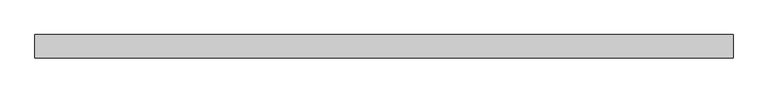
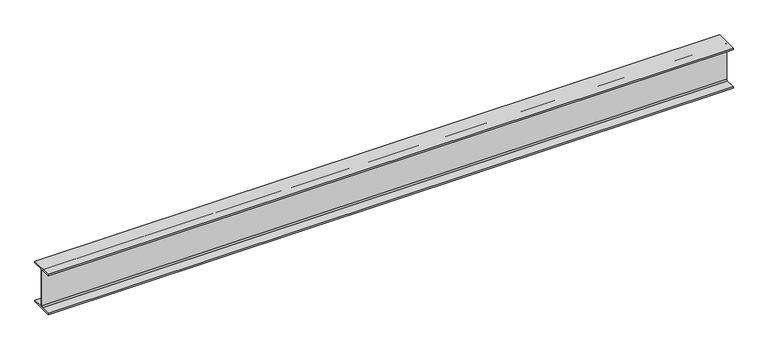
"""IFC4 building model written with IfcOpenShell, lengths in millimetres: beam geometry, Steel Beam_H-KSD3502 : H_SB_ASB_H-300x300x10x15."""

import ifcopenshell
import ifcopenshell.guid

model = None  # the IFC model being written
_history = None  # IfcOwnerHistory: only IFC2X3 demands one
_inside = {}  # id of a spatial element -> (the spatial element, [elements in it])
_under = {}  # id of a project, library or spatial element -> (it, [spatial elements below it])
_declared = {}  # id of a project -> (the project, [libraries it declares])
_typed = {}  # id of a type object -> (the type object, [elements of that type])
_made_of = {}  # id of a material, layer set ... -> (it, [elements and type objects made of it])


def new_model(schema):
    """Start an empty IFC model of exactly this schema.

    Asked for "IFC4X3", IfcOpenShell would pick the latest addendum, in which some entities
    have other attributes; the version numbers below select the first issue.
    IFC2X3 requires an IfcOwnerHistory on every rooted entity: one is made here for all.
    """
    global model, _history
    if schema == "IFC4X3":
        model = ifcopenshell.file(schema_version=(4, 3, 0, 0))
    else:
        model = ifcopenshell.file(schema=schema)
    _inside.clear()
    _under.clear()
    _declared.clear()
    _typed.clear()
    _made_of.clear()
    _history = None
    if model.schema == "IFC2X3":
        org = make("IfcOrganization", Name="unknown")
        user = make(
            "IfcPersonAndOrganization",
            ThePerson=make("IfcPerson", FamilyName="unknown"),
            TheOrganization=org,
        )
        app = make(
            "IfcApplication",
            ApplicationDeveloper=org,
            Version="unknown",
            ApplicationFullName="unknown",
            ApplicationIdentifier="unknown",
        )
        _history = make(
            "IfcOwnerHistory",
            OwningUser=user,
            OwningApplication=app,
            ChangeAction="ADDED",
            CreationDate=0,
        )
    return model


def make(cls, **values):
    """One entity of the class cls with the attributes given. An attribute that is None is left unset."""
    return model.create_entity(
        cls, **{name: value for name, value in values.items() if value is not None}
    )


def rooted(cls, **values):
    """An entity with a GlobalId (a new one), such as an element, a storey or a relation."""
    return make(cls, GlobalId=ifcopenshell.guid.new(), OwnerHistory=_history, **values)


def si_unit(unit_type, name, prefix=None):
    """IfcSIUnit, for example si_unit("LENGTHUNIT", "METRE", prefix="MILLI")."""
    return make("IfcSIUnit", UnitType=unit_type, Prefix=prefix, Name=name)


def assignment(units):
    """IfcUnitAssignment: the units of a project."""
    return None if units is None else make("IfcUnitAssignment", Units=units)


def point(xyz):
    """IfcCartesianPoint."""
    return None if xyz is None else make("IfcCartesianPoint", Coordinates=xyz)


def direction(xyz):
    """IfcDirection."""
    return None if xyz is None else make("IfcDirection", DirectionRatios=xyz)


def frame(location, z_axis=None, x_axis=None):
    """IfcAxis2Placement3D, a coordinate frame: its origin and axes. An axis left out is left unset."""
    return make(
        "IfcAxis2Placement3D",
        Location=point(location),
        Axis=direction(z_axis),
        RefDirection=direction(x_axis),
    )


def frame_2d(location, x_axis=None):
    """IfcAxis2Placement2D, a coordinate frame in the plane: its origin and x axis."""
    return make(
        "IfcAxis2Placement2D", Location=point(location), RefDirection=direction(x_axis)
    )


def origin():
    """The frame at (0, 0, 0) with its axes left unset."""
    return frame((0.0, 0.0, 0.0))


def place(relative_to, where):
    """IfcLocalPlacement: puts the frame where relative to a parent placement (None: the world)."""
    return make(
        "IfcLocalPlacement", PlacementRelTo=relative_to, RelativePlacement=where
    )


def context(
    kind, dimensions, precision=None, world=None, true_north=None, identifier=None
):
    """IfcGeometricRepresentationContext, for example the 3D "Model" context."""
    return make(
        "IfcGeometricRepresentationContext",
        ContextIdentifier=identifier,
        ContextType=kind,
        CoordinateSpaceDimension=dimensions,
        Precision=precision,
        WorldCoordinateSystem=world,
        TrueNorth=true_north,
    )


def project(units=None, contexts=None):
    """IfcProject with its units and contexts."""
    return rooted(
        "IfcProject",
        Name="project",
        RepresentationContexts=contexts,
        UnitsInContext=assignment(units),
    )


def spatial(cls, under=None, at=None, **own):
    """A site, building, storey or space (cls), placed at a placement, below another one or the project."""
    s = rooted(cls, ObjectPlacement=at, **own)
    if under is not None:
        _under.setdefault(under.id(), (under, []))[1].append(s)
    return s


def polyline(points):
    """IfcPolyline through the points."""
    return make("IfcPolyline", Points=[point(p) for p in points])


def circle_curve(where, radius):
    """IfcCircle in the frame where."""
    return make("IfcCircle", Position=where, Radius=radius)


def trimmed(basis, trim1, trim2, sense, master):
    """IfcTrimmedCurve: the piece of a basis curve between two trims."""
    return make(
        "IfcTrimmedCurve",
        BasisCurve=basis,
        Trim1=trim1,
        Trim2=trim2,
        SenseAgreement=sense,
        MasterRepresentation=master,
    )


def segment(curve, same_sense, transition):
    """IfcCompositeCurveSegment."""
    return make(
        "IfcCompositeCurveSegment",
        Transition=transition,
        SameSense=same_sense,
        ParentCurve=curve,
    )


def composite_curve(segments, self_intersect=None):
    """IfcCompositeCurve: segments joined end to end."""
    return make("IfcCompositeCurve", Segments=segments, SelfIntersect=self_intersect)


def outline(outer, holes=None, kind="AREA"):
    """IfcArbitraryClosedProfileDef: a profile drawn as a closed curve; with holes, ...WithVoids."""
    if holes is None:
        return make("IfcArbitraryClosedProfileDef", ProfileType=kind, OuterCurve=outer)
    return make(
        "IfcArbitraryProfileDefWithVoids",
        ProfileType=kind,
        OuterCurve=outer,
        InnerCurves=holes,
    )


def extrude(swept, where, along, depth):
    """IfcExtrudedAreaSolid: the profile swept, set in the frame where, extruded along a direction by depth."""
    return make(
        "IfcExtrudedAreaSolid",
        SweptArea=swept,
        Position=where,
        ExtrudedDirection=direction(along),
        Depth=depth,
    )


def shape(context_of_items, identifier, shape_type, items):
    """IfcShapeRepresentation: the items that make up one representation, for example the "Body"."""
    return make(
        "IfcShapeRepresentation",
        ContextOfItems=context_of_items,
        RepresentationIdentifier=identifier,
        RepresentationType=shape_type,
        Items=items,
    )


def source(mapping_origin, context_of_items, identifier, shape_type, items):
    """IfcRepresentationMap: a shape defined once, which mapped items show again and again."""
    return make(
        "IfcRepresentationMap",
        MappingOrigin=mapping_origin,
        MappedRepresentation=shape(context_of_items, identifier, shape_type, items),
    )


def transform(
    local_origin,
    x_axis=None,
    y_axis=None,
    z_axis=None,
    scale=None,
    scale2=None,
    scale3=None,
    uniform=True,
):
    """IfcCartesianTransformationOperator3D, or its non-uniform kind. x_axis, y_axis, z_axis: its Axis1, 2, 3."""
    if uniform:
        return make(
            "IfcCartesianTransformationOperator3D",
            Axis1=direction(x_axis),
            Axis2=direction(y_axis),
            LocalOrigin=point(local_origin),
            Scale=scale,
            Axis3=direction(z_axis),
        )
    return make(
        "IfcCartesianTransformationOperator3DnonUniform",
        Axis1=direction(x_axis),
        Axis2=direction(y_axis),
        LocalOrigin=point(local_origin),
        Scale=scale,
        Axis3=direction(z_axis),
        Scale2=scale2,
        Scale3=scale3,
    )


def mapped(mapping_source, mapping_target):
    """IfcMappedItem: shows the shape of a source again, moved by a transform."""
    return make(
        "IfcMappedItem", MappingSource=mapping_source, MappingTarget=mapping_target
    )


def made_of(thing, what):
    """Note that an element or type object is made of a material, layer set ...; save() writes the relation."""
    if what is not None:
        _made_of.setdefault(what.id(), (what, []))[1].append(thing)
    return thing


def element(
    cls,
    number,
    at=None,
    inside=None,
    cuts=None,
    type_object=None,
    material=None,
    context=None,
    identifier="Body",
    shape_type=None,
    held_by="IfcProductDefinitionShape",
    body=None,
    shapes=None,
    **own,
):
    """One element of the class cls, such as IfcWall. Its Tag is "e" and its number.

    at: its placement. inside: the storey or other place that contains it. cuts: it is an
    opening in that element (IfcRelVoidsElement). A single representation is given by context,
    identifier, shape_type and body (its items); several are given by shapes. held_by: the class
    of the entity that holds the representations. save() writes the other relations.
    """
    e = rooted(cls, Tag="e%d" % number, ObjectPlacement=at, **own)
    if body is not None:
        shapes = [shape(context, identifier, shape_type, body)]
    if shapes is not None:
        e.Representation = make(held_by, Representations=shapes)
    if inside is not None:
        _inside.setdefault(inside.id(), (inside, []))[1].append(e)
    if cuts is not None:
        rooted(
            "IfcRelVoidsElement", RelatingBuildingElement=cuts, RelatedOpeningElement=e
        )
    if type_object is not None:
        _typed.setdefault(type_object.id(), (type_object, []))[1].append(e)
    return made_of(e, material)


def aggregate(whole, parts):
    """IfcRelAggregates: a whole, such as a stair, and the parts it consists of."""
    return rooted("IfcRelAggregates", RelatingObject=whole, RelatedObjects=parts)


def save(model, path):
    """Write the relations noted so far, then the file.

    IfcRelAggregates (storeys below a building ...), IfcRelContainedInSpatialStructure (elements
    in a storey), IfcRelDefinesByType, IfcRelAssociatesMaterial and IfcRelDeclares: one each for
    every whole, place, type object, material and project.
    """
    for whole, parts in _under.values():
        aggregate(whole, parts)
    for where, things in _inside.values():
        rooted(
            "IfcRelContainedInSpatialStructure",
            RelatedElements=things,
            RelatingStructure=where,
        )
    for kind, things in _typed.values():
        rooted("IfcRelDefinesByType", RelatedObjects=things, RelatingType=kind)
    for what, things in _made_of.values():
        rooted("IfcRelAssociatesMaterial", RelatedObjects=things, RelatingMaterial=what)
    for by, libraries in _declared.values():
        rooted("IfcRelDeclares", RelatingContext=by, RelatedDefinitions=libraries)
    model.write(path)


def beam_952dd806(model_context):
    return source(origin(), model_context, "Body", "SweptSolid", [
        extrude(outline(composite_curve([segment(polyline([(-82.5, -141.5), (-11.9, -141.5)]), True, "CONTINUOUS"), segment(trimmed(circle_curve(frame_2d((-11.9, -132.6)), 8.9), [point((-11.9, -141.5))], [point((-3.0, -132.6))], True, "CARTESIAN"), True, "CONTINUOUS"), segment(polyline([(-3.0, -132.6), (-3.0, 132.6)]), True, "CONTINUOUS"), segment(trimmed(circle_curve(frame_2d((-11.9, 132.6)), 8.9), [point((-3.0, 132.6))], [point((-11.9, 141.5))], True, "CARTESIAN"), True, "CONTINUOUS"), segment(polyline([(-11.9, 141.5), (-82.5, 141.5), (-82.5, 151.7), (82.5, 151.7), (82.5, 141.5), (11.9, 141.5)]), True, "CONTINUOUS"), segment(trimmed(circle_curve(frame_2d((11.9, 132.6)), 8.9), [point((11.9, 141.5))], [point((3.0, 132.6))], True, "CARTESIAN"), True, "CONTINUOUS"), segment(polyline([(3.0, 132.6), (3.0, -132.6)]), True, "CONTINUOUS"), segment(trimmed(circle_curve(frame_2d((11.9, -132.6)), 8.9), [point((3.0, -132.6))], [point((11.9, -141.5))], True, "CARTESIAN"), True, "CONTINUOUS"), segment(polyline([(11.9, -141.5), (82.5, -141.5), (82.5, -151.7), (-82.5, -151.7), (-82.5, -141.5)]), True, "CONTINUOUS")], self_intersect=False)), frame((-2479.7628546, 0.0, 0.0), z_axis=(1.0, 0.0, 0.0), x_axis=(0.0, 1.0, 0.0)), (0.0, 0.0, 1.0), 4891.0868037),
    ])


if __name__ == "__main__":
    model = new_model("IFC4")
    model_context = context("Model", 3, world=origin())
    ifc_project = project(units=[si_unit("LENGTHUNIT", "METRE", prefix="MILLI")], contexts=[model_context])
    site = spatial("IfcSite", under=ifc_project)
    building = spatial("IfcBuilding", under=site)
    placement = place(None, origin())
    beam_shape = beam_952dd806(model_context)
    element("IfcBeam", 1, ObjectType="Steel Beam_H-KSD3502 : H_SB_ASB_H-300x300x10x15", at=placement, inside=building, context=model_context, shape_type="MappedRepresentation", body=[
        mapped(beam_shape, transform((0.0, 0.0, 0.0), x_axis=(1.0, 0.0, 0.0), y_axis=(0.0, 1.0, 0.0), z_axis=(0.0, 0.0, 1.0))),
    ])
    save(model, "model.ifc")

# Revit data of these elements
# Type "Steel Beam_H-KSD3502 : H_SB_ASB_H-300x300x10x15"
#   Width = 30.0 cm
#   Web Thickness = 1.0 cm
#   Web Fillet = 1.8 cm
#   Warping Constant = 1370670.0 cm⁶
#   Torsional Moment of Inertia = 77.00 cm⁴
#   Torsional Modulus = 1.0 cm³
#   Section Area = 119.8 cm²
#   Plastic Modulus weak axis = 684.0 cm³
#   Plastic Modulus strong axis = 1500.0 cm³
#   Perimeter = 1.75 m²/m
#   Nominal Weight = 94.00 kgf/m
#   Moment of Inertia weak axis = 6750.00 cm⁴
#   Moment of Inertia strong axis = 20400.00 cm⁴
#   Height = 30.0 cm
#   Flange Thickness = 1.5 cm
#   Elastic Modulus weak axis = 450.0 cm³
#   Elastic Modulus strong axis = 1360.0 cm³
#   Centroid Vertical = 15.0 cm
#   Centroid Horizontal = 15.0 cm
#   Length [instance default] = 1.5240 m
#   Structural Material [instance default] = Steel, 45-345
#   Assembly Code = ""
# Element 1 (IfcBeam, "Steel Beam_H-KSD3502 : H_SB_ASB_H-300x300x10x15")
#   Structural Material = none
# Materials
#   "Steel, 45-345": class "Metal", colour RGB 189 187 185, transparency 0, Description = "Steel 345 MPa", Cost = 0
